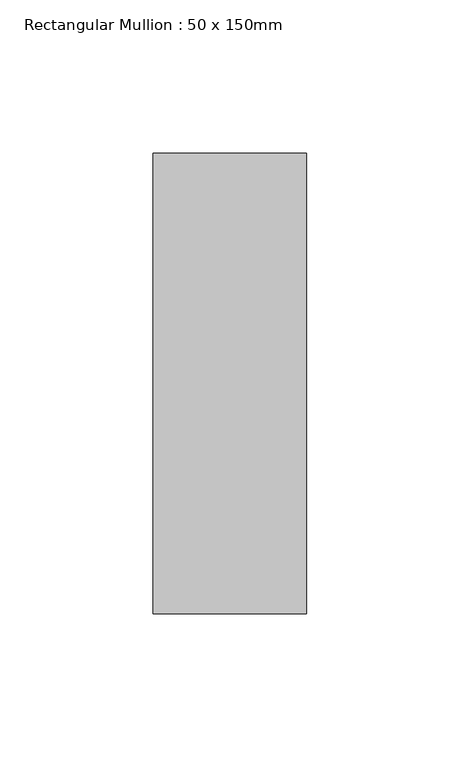
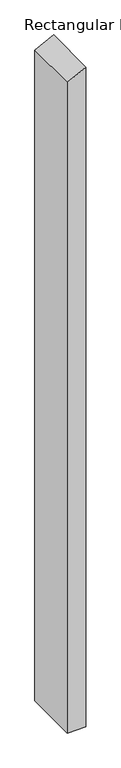
"""IFC4 building model written with IfcOpenShell, lengths in millimetres: member geometry, Rectangular Mullion : 50 x 150mm."""

from ifc_helpers import new_model, si_unit, frame, origin, place, context, project, spatial, polyline, outline, extrude, source, transform, mapped, element, save


def rectangular_mullion_50_x_150mm_278098da(model_context):
    return source(origin(), model_context, "Body", "SweptSolid", [
        extrude(outline(polyline([(0.0, 0.0), (-26.0283525, -50.0), (-1870.0207538, -50.0), (-1870.0207538, 0.0), (0.0, 0.0)])), frame((0.0, -75.0, 0.0), z_axis=(0.0, 1.0, 0.0), x_axis=(0.0, 0.0, 1.0)), (0.0, 0.0, 1.0), 150.0),
    ])


if __name__ == "__main__":
    model = new_model("IFC4")
    model_context = context("Model", 3, world=origin())
    ifc_project = project(units=[si_unit("LENGTHUNIT", "METRE", prefix="MILLI")], contexts=[model_context])
    site = spatial("IfcSite", under=ifc_project)
    building = spatial("IfcBuilding", under=site)
    placement = place(None, origin())
    rectangular_mullion_50_x_150mm_shape = rectangular_mullion_50_x_150mm_278098da(model_context)
    element("IfcMember", 1, ObjectType="Rectangular Mullion : 50 x 150mm", at=placement, inside=building, context=model_context, shape_type="MappedRepresentation", body=[
        mapped(rectangular_mullion_50_x_150mm_shape, transform((0.0, 0.0, 0.0), x_axis=(1.0, 0.0, 0.0), y_axis=(0.0, 1.0, 0.0), z_axis=(0.0, 0.0, 1.0))),
    ])
    save(model, "model.ifc")

# Revit data of these elements
# Type "Rectangular Mullion : 50 x 150mm"
#   built-in parameter 1007304 = 0.492126 (stored number, unit not read)
#   built-in parameter 1007301 = 0.082021 (stored number, unit not read)
#   built-in parameter 1007300 = 0.082021 (stored number, unit not read)
# Element 1 (IfcMember, "Rectangular Mullion : 50 x 150mm")
#   Materials on its faces: "Aluminium"
# Materials
#   "Aluminium": class "Metal", colour RGB 247 247 247, transparency 0, Description = "Aluminium 6061", Cost = 0
